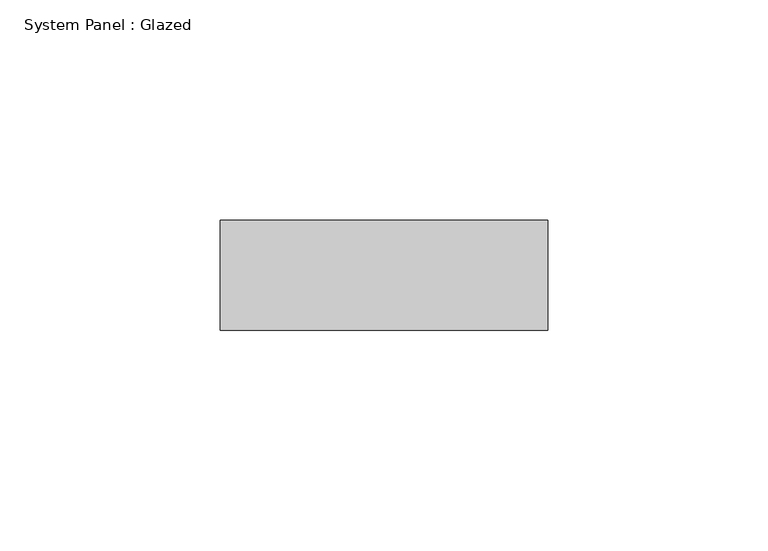
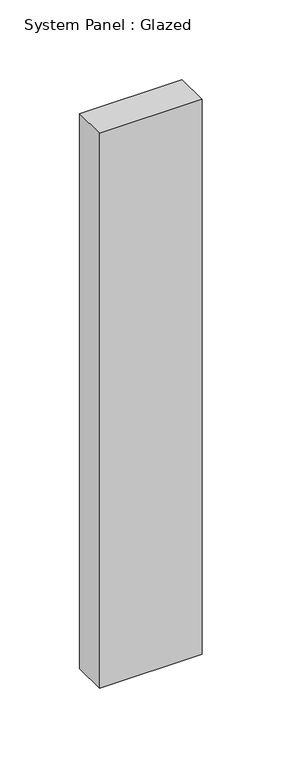
"""IFC4 building model written with IfcOpenShell, lengths in millimetres: plate geometry, System Panel : Glazed."""

from ifc_helpers import new_model, si_unit, origin, origin_with_axes, place, context, project, spatial, polyline, outline, extrude, source, transform, mapped, element, save


def system_panel_glazed_e987ce54(model_context):
    return source(origin(), model_context, "Body", "SweptSolid", [
        extrude(outline(polyline([(37.2092572, 24.5), (-37.2092572, 24.5), (-37.2092572, 49.5), (37.2092572, 49.5), (37.2092572, 24.5)])), origin_with_axes(), (0.0, 0.0, 1.0), 425.0),
    ])


if __name__ == "__main__":
    model = new_model("IFC4")
    model_context = context("Model", 3, world=origin())
    ifc_project = project(units=[si_unit("LENGTHUNIT", "METRE", prefix="MILLI")], contexts=[model_context])
    site = spatial("IfcSite", under=ifc_project)
    building = spatial("IfcBuilding", under=site)
    placement = place(None, origin())
    system_panel_glazed_shape = system_panel_glazed_e987ce54(model_context)
    element("IfcPlate", 1, ObjectType="System Panel : Glazed", at=placement, inside=building, context=model_context, shape_type="MappedRepresentation", body=[
        mapped(system_panel_glazed_shape, transform((0.0, 0.0, 0.0), x_axis=(1.0, 0.0, 0.0), y_axis=(0.0, 1.0, 0.0), z_axis=(0.0, 0.0, 1.0))),
    ])
    save(model, "model.ifc")

# Revit data of these elements
# Type "System Panel : Glazed"
#   Keynote = "H11"
#   Construction Type Id = "GSP4R"
#   Analytic Construction = "1/8 in Pilkington single glazing"
#   Visual Light Transmittance = 0.9
#   Solar Heat Gain Coefficient = 0.86
#   Heat Transfer Coefficient (U) = 6.7069 W/(m²·K)
# Element 1 (IfcPlate, "System Panel : Glazed")
#   Materials on its faces: "Glass"
# Materials
#   "Glass": class "Glass", colour RGB 0 128 192, transparency 0.9, Description = "Soda Lime Glass", Cost = 0
